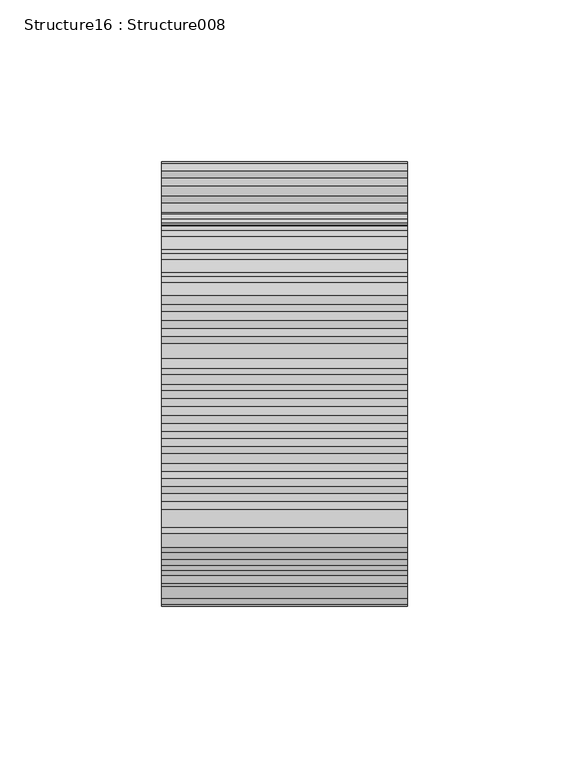
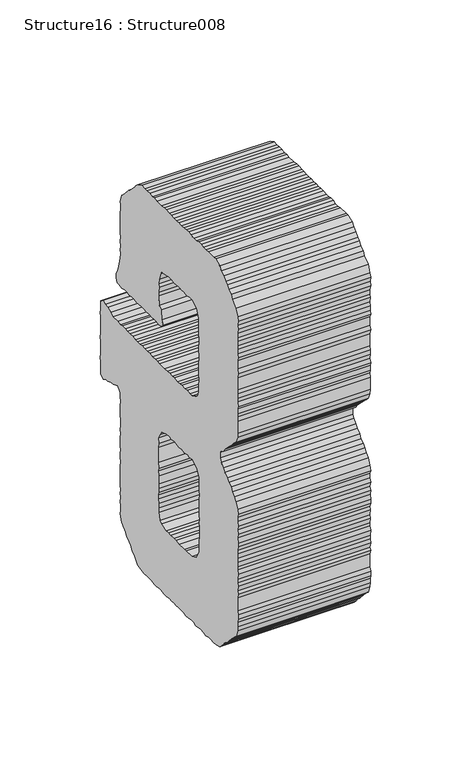
"""IFC4 building model written with IfcOpenShell, lengths in millimetres: proxy geometry, Structure16 : Structure008."""

from ifc_helpers import new_model, si_unit, frame, origin, place, context, project, spatial, polyline, outline, extrude, source, transform, mapped, element, save


def structure16_structure008_b6baecb6(model_context):
    return source(origin(), model_context, "Body", "SweptSolid", [
        extrude(outline(polyline([(4.9551582, 0.0), (7.1061493, 0.6235248), (9.2842501, 0.3176927), (12.0604604, 0.3176927), (14.2385612, 0.0), (17.0156186, 0.3176927), (18.8633191, 0.0), (21.6624032, 0.0), (24.4377663, 0.6235248), (26.9115331, 0.3176927), (29.3929245, 0.6235248), (31.8658442, 0.0), (35.8874096, -1.8587138), (38.9719935, -5.5651282), (41.4533849, -6.4953323), (42.9935589, -8.9657104), (44.8548143, -10.5075787), (46.1010167, -12.0604604), (48.2562437, -13.9191743), (50.1259709, -16.0845674), (52.2786563, -17.6374491), (53.831538, -21.9673882), (53.5282474, -23.8150887), (53.5282474, -29.3920774), (53.2063189, -31.8633027), (53.2063189, -34.3345279), (53.831538, -36.4990739), (53.831538, -38.9702992), (53.2063189, -41.1467057), (53.2063189, -43.6179309), (53.5282474, -46.7008205), (53.831538, -48.877227), (53.5282474, -51.3484523), (53.5282474, -53.5248587), (53.2063189, -55.996084), (53.5282474, -58.4673093), (53.2063189, -61.25538), (53.2063189, -63.7266053), (53.5282474, -66.1978306), (53.5282474, -68.0565444), (53.831538, -71.1512945), (53.831538, -73.0100083), (53.2063189, -76.1047584), (53.2063189, -80.7405296), (53.831538, -82.9059228), (53.2063189, -85.3890086), (53.831538, -87.8593867), (53.5282474, -90.6364441), (53.5282474, -92.8018372), (53.831538, -95.589908), (51.65259, -99.614015), (50.1259709, -101.4617155), (48.2562437, -102.6969045), (44.2431501, -106.7210115), (42.9935589, -108.5805725), (41.4533849, -109.8157615), (37.124293, -113.8398685), (35.5697169, -115.6985824), (31.2414722, -116.9346186), (29.085398, -116.6287865), (26.9115331, -116.6287865), (24.1353229, -116.9346186), (21.3447106, -116.9346186), (18.8633191, -117.2523112), (13.9225629, -117.2523112), (12.0604604, -116.9346186), (9.5875407, -116.6287865), (7.1061493, -116.9346186), (4.0266485, -116.6287865), (1.8612553, -117.2523112), (-0.9285098, -116.6287865), (-3.0930557, -116.9346186), (-7.7305213, -118.1698076), (-12.6848324, -119.4049967), (-15.1535162, -120.9587256), (-17.9432813, -121.2526972), (-20.4263671, -120.0285215), (-20.4263671, -118.1698076), (-20.7330464, -115.3808897), (-20.1086744, -112.6046795), (-20.1086744, -110.1215937), (-20.7330464, -107.9680611), (-20.1086744, -105.1799903), (-20.1086744, -103.0145972), (-20.7330464, -100.5433719), (-20.1086744, -95.589908), (-20.1086744, -93.425362), (-20.4263671, -90.9422762), (-20.1086744, -88.1652188), (-20.7330464, -85.3890086), (-20.1086744, -83.2117549), (-20.1086744, -81.0472089), (-20.7330464, -78.5759837), (-20.1086744, -76.1047584), (-18.247419, -73.9283519), (-15.7787353, -75.4812336), (-10.1992051, -76.4105905), (-8.3565877, -77.9524589), (-3.0930557, -78.5759837), (-0.9285098, -78.5759837), (2.4813914, -77.9524589), (4.3299391, -78.5759837), (7.1061493, -78.258291), (11.4360884, -76.7164227), (12.9889701, -75.4812336), (13.9225629, -70.8336018), (14.542699, -68.6800692), (14.2385612, -65.8801379), (13.9225629, -63.1030805), (14.2385612, -61.25538), (14.542699, -58.1496166), (14.2385612, -55.6783914), (14.542699, -53.5248587), (13.9225629, -50.7249275), (14.542699, -47.9478701), (14.542699, -45.4766448), (12.0604604, -40.829013), (7.1061493, -38.9702992), (-2.164546, -38.9702992), (-5.2491299, -38.3586349), (-7.4229949, -38.3586349), (-9.8950673, -38.6644671), (-12.3781531, -38.6644671), (-14.8502256, -38.3586349), (-17.0012166, -38.3586349), (-20.1086744, -38.9702992), (-22.2732204, -38.9702992), (-24.4386135, -38.6644671), (-27.2283786, -38.6644671), (-29.3793697, -38.3586349), (-34.334528, -38.9702992), (-37.4275837, -38.9702992), (-40.5341943, -39.8996561), (-42.0650493, -42.0650492), (-43.617931, -45.1708127), (-44.2439973, -47.9478701), (-43.617931, -50.4190953), (-43.9356236, -52.5836413), (-43.617931, -55.6783914), (-43.9356236, -57.5379524), (-44.2439973, -60.0083305), (-43.617931, -63.1030805), (-43.9356236, -64.9617944), (-43.617931, -67.7507123), (-43.9356236, -70.2219376), (-44.2439973, -73.0100083), (-44.2439973, -77.9524589), (-43.9356236, -80.1170048), (-43.9356236, -82.282398), (-44.2439973, -85.3890086), (-43.617931, -87.8593867), (-43.9356236, -90.0129193), (-43.9356236, -92.4951579), (-43.617931, -94.9663832), (-44.2439973, -97.7434406), (-43.9356236, -99.9198471), (-44.2439973, -102.0852402), (-43.617931, -104.5564655), (-43.617931, -107.3445363), (-43.9356236, -110.1215937), (-43.617931, -112.2980002), (-43.617931, -115.0750576), (-44.2439973, -117.2523112), (-43.617931, -119.7226893), (-43.617931, -124.3593078), (-42.0650493, -126.5238537), (-41.1365395, -129.6067433), (-40.8281659, -132.0898291), (-39.5921296, -134.254375), (-41.1365395, -136.4197682), (-46.7109867, -136.4197682), (-48.5722421, -137.0314324), (-51.0409258, -136.7374608), (-54.1348287, -136.4197682), (-56.3044577, -136.7374608), (-59.0891398, -136.4197682), (-60.9368402, -136.7374608), (-63.4190789, -137.0314324), (-65.8919985, -136.4197682), (-70.8463096, -136.4197682), (-73.6225198, -136.7374608), (-75.7963848, -137.0314324), (-78.8809687, -136.4197682), (-86.0006729, -136.4197682), (-87.5535546, -134.254375), (-86.3081994, -131.7831498), (-86.0006729, -129.3009111), (-84.7544705, -126.5238537), (-84.446944, -124.0526284), (-82.90677, -119.7226893), (-85.3754537, -116.9346186), (-87.8568452, -116.9346186), (-90.3297648, -116.6287865), (-93.4236677, -116.9346186), (-95.5882137, -116.9346186), (-98.3779788, -117.2523112), (-102.7079179, -116.6287865), (-105.1808375, -116.6287865), (-107.9655195, -117.2523112), (-110.1351486, -116.6287865), (-112.2861397, -116.9346186), (-115.3935974, -117.2523112), (-117.5445885, -116.9346186), (-120.3343536, -116.6287865), (-122.195609, -117.2523112), (-124.6642927, -116.9346186), (-127.4540579, -116.6287865), (-129.6186038, -117.2523112), (-132.394814, -116.9346186), (-136.7247532, -116.9346186), (-139.2061446, -117.2523112), (-141.9967569, -117.2523112), (-144.4688294, -116.6287865), (-146.6342225, -117.2523112), (-149.1020591, -116.6287865), (-151.5842977, -116.9346186), (-154.3647438, -116.6287865), (-156.5301369, -116.6287865), (-159.314819, -117.2523112), (-163.6354391, -115.6985824), (-164.8816415, -113.8398685), (-167.0461875, -111.6744754), (-169.2107334, -110.4392863), (-170.7644623, -107.9680611), (-171.9869437, -106.4151794), (-174.4734182, -105.1799903), (-176.3304376, -102.6969045), (-177.5664739, -101.4617155), (-180.0351576, -99.614015), (-180.9679033, -95.2722153), (-181.2711938, -93.1195299), (-180.9679033, -90.330612), (-180.9679033, -85.9888123), (-181.5888865, -83.2117549), (-181.5888865, -80.7405296), (-180.9679033, -78.258291), (-180.9679033, -76.1047584), (-181.5888865, -73.6343803), (-181.5888865, -70.5277697), (-180.9679033, -68.3623766), (-181.2711938, -65.8801379), (-180.9679033, -63.1030805), (-181.2711938, -61.25538), (-180.9679033, -58.4673093), (-180.9679033, -53.8315381), (-181.5888865, -51.6542844), (-181.2711938, -48.5713948), (-180.9679033, -46.3949884), (-180.9679033, -43.9237631), (-181.5888865, -41.7702305), (-180.9679033, -36.8167666), (-180.9679033, -33.7220165), (-181.5888865, -31.54561), (-180.9679033, -28.7685526), (-180.9679033, -26.9098388), (-181.2711938, -23.8150887), (-180.9679033, -21.3438634), (-179.731867, -17.6374491), (-178.191693, -15.7787353), (-176.0135922, -13.6133421), (-174.4734182, -12.6839852), (-172.6121628, -10.2127599), (-171.0719888, -8.9657104), (-168.5905974, -6.8011644), (-167.3630329, -5.5651282), (-164.8816415, -3.0828895), (-163.6354391, -1.5528817), (-159.314819, 0.0), (-156.8334275, 0.3176927), (-154.0572173, 0.3176927), (-152.2001978, 0.6235248), (-149.4104327, 0.6235248), (-147.2543586, 0.0), (-139.2061446, 0.0), (-136.7247532, 0.6235248), (-135.1845792, 0.0), (-132.0872876, 0.6235248), (-129.9218944, 0.3176927), (-127.7709033, 0.3176927), (-124.6642927, 0.6235248), (-122.195609, 0.0), (-120.3343536, 0.0), (-117.5445885, 0.3176927), (-115.3935974, 0.0), (-112.2861397, 0.3176927), (-110.4384392, 0.0), (-107.9655195, 0.6235248), (-105.7916546, 0.6235248), (-102.7079179, 0.3176927), (-100.2256793, 0.6235248), (-98.0611333, 0.0), (-95.2849231, 0.6235248), (-92.8026844, 0.0), (-90.3297648, 0.0), (-88.1652188, 0.6235248), (-85.3754537, 0.0), (-81.9740244, -1.8587138), (-79.8094784, -3.4005822), (-77.9524589, -5.259296), (-75.7963848, -6.4953323), (-74.5510295, -8.9657104), (-72.4000385, -10.2127599), (-70.5294641, -12.6839852), (-68.6682087, -14.2368669), (-66.5172177, -16.0845674), (-64.6466433, -17.3197564), (-61.2452139, -17.3197564), (-60.0176495, -16.0845674), (-58.4690037, -13.9191743), (-56.6077483, -12.6839852), (-54.4432024, -10.8252714), (-51.0409258, -7.1069965), (-48.8670608, -4.9534639), (-47.6394964, -3.7064143), (-45.7824769, -1.8587138), (-41.7566756, 0.0), (-38.9804654, 0.3176927), (-31.5574706, 0.3176927), (-29.0760791, 0.0), (-27.2283786, 0.3176927), (-24.1302399, 0.3176927), (-22.5815941, 0.6235248), (-20.1086744, 0.0), (-17.627283, 0.3176927), (-14.8502256, 0.3176927), (-12.6848324, 0.0), (-5.2491299, 0.0), (-2.4729197, 0.6235248), (0.0, 0.0), (4.9551582, 0.0)]), holes=[polyline([(-84.446944, -75.4812336), (-82.90677, -71.1512945), (-82.90677, -68.3623766), (-83.2100606, -66.5036627), (-82.90677, -63.4089127), (-83.2100606, -60.6318553), (-83.5277532, -58.4673093), (-82.90677, -55.996084), (-83.5277532, -53.5248587), (-82.90677, -50.4190953), (-83.2100606, -48.5713948), (-82.90677, -45.4766448), (-85.0721631, -41.1467057), (-89.7045457, -38.9702992), (-92.8026844, -38.9702992), (-94.9680776, -38.6644671), (-97.4359141, -38.9702992), (-100.2256793, -38.3586349), (-102.7079179, -38.9702992), (-107.3453835, -38.9702992), (-109.81322, -38.6644671), (-112.6038323, -38.9702992), (-114.7683783, -38.3586349), (-117.5445885, -38.9702992), (-119.4151629, -38.3586349), (-124.6642927, -38.3586349), (-129.6186038, -38.9702992), (-132.394814, -38.9702992), (-134.8770527, -38.6644671), (-138.5860085, -40.5231809), (-139.8178089, -41.4525378), (-141.6790642, -45.4766448), (-141.6790642, -51.0426201), (-141.9967569, -52.901334), (-141.9967569, -58.1496166), (-141.3715377, -61.25538), (-141.6790642, -63.4089127), (-141.6790642, -66.5036627), (-141.3715377, -68.6800692), (-141.6790642, -71.1512945), (-140.1261825, -75.4812336), (-138.902854, -77.0341153), (-134.5737621, -77.9524589), (-132.0872876, -78.258291), (-129.3017583, -78.258291), (-126.8288387, -78.5759837), (-124.3610022, -78.5759837), (-122.4988996, -78.258291), (-120.0175082, -77.9524589), (-117.2412979, -78.258291), (-112.6038323, -78.258291), (-109.5099294, -78.5759837), (-107.662229, -77.9524589), (-104.5556184, -78.5759837), (-95.2849231, -78.5759837), (-92.495158, -77.9524589), (-89.7045457, -78.5759837), (-86.3081994, -76.7164227), (-84.446944, -75.4812336)])]), frame((-35624.0862846, 277779.326112, 4164.4093762), z_axis=(1.0, 0.0, 1.354250045437766e-12), x_axis=(-1.354250045437766e-12, 0.0, 1.0)), (0.0, 0.0, 1.0), 76.2),
    ])


if __name__ == "__main__":
    model = new_model("IFC4")
    model_context = context("Model", 3, world=origin())
    ifc_project = project(units=[si_unit("LENGTHUNIT", "METRE", prefix="MILLI")], contexts=[model_context])
    site = spatial("IfcSite", under=ifc_project)
    building = spatial("IfcBuilding", under=site)
    placement = place(None, origin())
    structure16_structure008_shape = structure16_structure008_b6baecb6(model_context)
    element("IfcBuildingElementProxy", 1, Name="Structure16 : Structure008", ObjectType="Structure16 : Structure008", at=placement, inside=building, context=model_context, shape_type="MappedRepresentation", body=[
        mapped(structure16_structure008_shape, transform((0.0, 0.0, 0.0), x_axis=(1.0, 0.0, 0.0), y_axis=(0.0, 1.0, 0.0), z_axis=(0.0, 0.0, 1.0))),
    ])
    save(model, "model.ifc")

# Revit data of these elements
# Type "Structure16 : Structure008"
#   NameOverride = "Structure008"
# Element 1 (IfcBuildingElementProxy, "Structure16 : Structure008")
#   Materials on its faces: "BRUSHED ALUMINUM LETTERING"
# Materials
#   "BRUSHED ALUMINUM LETTERING": class "Unassigned", colour RGB 169 181 186, transparency 0, Cost = 0
